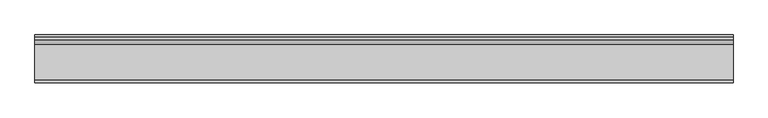
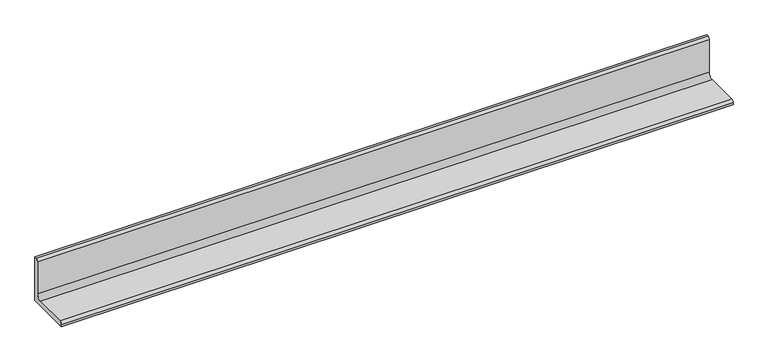
"""IFC4 building model written with IfcOpenShell, lengths in millimetres: beam geometry, NLRS_28_SF_LIB_stalen ligger hoekprofiel gelijkzijdig-AV-MMBS-SRP_gen_rsf : stalen ligger gelijkzijdig hoekprofiel LEQU_gen__150x150x15."""

import ifcopenshell
import ifcopenshell.guid

model = None  # the IFC model being written
_history = None  # IfcOwnerHistory: only IFC2X3 demands one
_inside = {}  # id of a spatial element -> (the spatial element, [elements in it])
_under = {}  # id of a project, library or spatial element -> (it, [spatial elements below it])
_declared = {}  # id of a project -> (the project, [libraries it declares])
_typed = {}  # id of a type object -> (the type object, [elements of that type])
_made_of = {}  # id of a material, layer set ... -> (it, [elements and type objects made of it])


def new_model(schema):
    """Start an empty IFC model of exactly this schema.

    Asked for "IFC4X3", IfcOpenShell would pick the latest addendum, in which some entities
    have other attributes; the version numbers below select the first issue.
    IFC2X3 requires an IfcOwnerHistory on every rooted entity: one is made here for all.
    """
    global model, _history
    if schema == "IFC4X3":
        model = ifcopenshell.file(schema_version=(4, 3, 0, 0))
    else:
        model = ifcopenshell.file(schema=schema)
    _inside.clear()
    _under.clear()
    _declared.clear()
    _typed.clear()
    _made_of.clear()
    _history = None
    if model.schema == "IFC2X3":
        org = make("IfcOrganization", Name="unknown")
        user = make(
            "IfcPersonAndOrganization",
            ThePerson=make("IfcPerson", FamilyName="unknown"),
            TheOrganization=org,
        )
        app = make(
            "IfcApplication",
            ApplicationDeveloper=org,
            Version="unknown",
            ApplicationFullName="unknown",
            ApplicationIdentifier="unknown",
        )
        _history = make(
            "IfcOwnerHistory",
            OwningUser=user,
            OwningApplication=app,
            ChangeAction="ADDED",
            CreationDate=0,
        )
    return model


def make(cls, **values):
    """One entity of the class cls with the attributes given. An attribute that is None is left unset."""
    return model.create_entity(
        cls, **{name: value for name, value in values.items() if value is not None}
    )


def rooted(cls, **values):
    """An entity with a GlobalId (a new one), such as an element, a storey or a relation."""
    return make(cls, GlobalId=ifcopenshell.guid.new(), OwnerHistory=_history, **values)


def si_unit(unit_type, name, prefix=None):
    """IfcSIUnit, for example si_unit("LENGTHUNIT", "METRE", prefix="MILLI")."""
    return make("IfcSIUnit", UnitType=unit_type, Prefix=prefix, Name=name)


def assignment(units):
    """IfcUnitAssignment: the units of a project."""
    return None if units is None else make("IfcUnitAssignment", Units=units)


def point(xyz):
    """IfcCartesianPoint."""
    return None if xyz is None else make("IfcCartesianPoint", Coordinates=xyz)


def direction(xyz):
    """IfcDirection."""
    return None if xyz is None else make("IfcDirection", DirectionRatios=xyz)


def frame(location, z_axis=None, x_axis=None):
    """IfcAxis2Placement3D, a coordinate frame: its origin and axes. An axis left out is left unset."""
    return make(
        "IfcAxis2Placement3D",
        Location=point(location),
        Axis=direction(z_axis),
        RefDirection=direction(x_axis),
    )


def frame_2d(location, x_axis=None):
    """IfcAxis2Placement2D, a coordinate frame in the plane: its origin and x axis."""
    return make(
        "IfcAxis2Placement2D", Location=point(location), RefDirection=direction(x_axis)
    )


def origin():
    """The frame at (0, 0, 0) with its axes left unset."""
    return frame((0.0, 0.0, 0.0))


def place(relative_to, where):
    """IfcLocalPlacement: puts the frame where relative to a parent placement (None: the world)."""
    return make(
        "IfcLocalPlacement", PlacementRelTo=relative_to, RelativePlacement=where
    )


def context(
    kind, dimensions, precision=None, world=None, true_north=None, identifier=None
):
    """IfcGeometricRepresentationContext, for example the 3D "Model" context."""
    return make(
        "IfcGeometricRepresentationContext",
        ContextIdentifier=identifier,
        ContextType=kind,
        CoordinateSpaceDimension=dimensions,
        Precision=precision,
        WorldCoordinateSystem=world,
        TrueNorth=true_north,
    )


def project(units=None, contexts=None):
    """IfcProject with its units and contexts."""
    return rooted(
        "IfcProject",
        Name="project",
        RepresentationContexts=contexts,
        UnitsInContext=assignment(units),
    )


def spatial(cls, under=None, at=None, **own):
    """A site, building, storey or space (cls), placed at a placement, below another one or the project."""
    s = rooted(cls, ObjectPlacement=at, **own)
    if under is not None:
        _under.setdefault(under.id(), (under, []))[1].append(s)
    return s


def polyline(points):
    """IfcPolyline through the points."""
    return make("IfcPolyline", Points=[point(p) for p in points])


def circle_curve(where, radius):
    """IfcCircle in the frame where."""
    return make("IfcCircle", Position=where, Radius=radius)


def trimmed(basis, trim1, trim2, sense, master):
    """IfcTrimmedCurve: the piece of a basis curve between two trims."""
    return make(
        "IfcTrimmedCurve",
        BasisCurve=basis,
        Trim1=trim1,
        Trim2=trim2,
        SenseAgreement=sense,
        MasterRepresentation=master,
    )


def segment(curve, same_sense, transition):
    """IfcCompositeCurveSegment."""
    return make(
        "IfcCompositeCurveSegment",
        Transition=transition,
        SameSense=same_sense,
        ParentCurve=curve,
    )


def composite_curve(segments, self_intersect=None):
    """IfcCompositeCurve: segments joined end to end."""
    return make("IfcCompositeCurve", Segments=segments, SelfIntersect=self_intersect)


def outline(outer, holes=None, kind="AREA"):
    """IfcArbitraryClosedProfileDef: a profile drawn as a closed curve; with holes, ...WithVoids."""
    if holes is None:
        return make("IfcArbitraryClosedProfileDef", ProfileType=kind, OuterCurve=outer)
    return make(
        "IfcArbitraryProfileDefWithVoids",
        ProfileType=kind,
        OuterCurve=outer,
        InnerCurves=holes,
    )


def extrude(swept, where, along, depth):
    """IfcExtrudedAreaSolid: the profile swept, set in the frame where, extruded along a direction by depth."""
    return make(
        "IfcExtrudedAreaSolid",
        SweptArea=swept,
        Position=where,
        ExtrudedDirection=direction(along),
        Depth=depth,
    )


def shape(context_of_items, identifier, shape_type, items):
    """IfcShapeRepresentation: the items that make up one representation, for example the "Body"."""
    return make(
        "IfcShapeRepresentation",
        ContextOfItems=context_of_items,
        RepresentationIdentifier=identifier,
        RepresentationType=shape_type,
        Items=items,
    )


def source(mapping_origin, context_of_items, identifier, shape_type, items):
    """IfcRepresentationMap: a shape defined once, which mapped items show again and again."""
    return make(
        "IfcRepresentationMap",
        MappingOrigin=mapping_origin,
        MappedRepresentation=shape(context_of_items, identifier, shape_type, items),
    )


def transform(
    local_origin,
    x_axis=None,
    y_axis=None,
    z_axis=None,
    scale=None,
    scale2=None,
    scale3=None,
    uniform=True,
):
    """IfcCartesianTransformationOperator3D, or its non-uniform kind. x_axis, y_axis, z_axis: its Axis1, 2, 3."""
    if uniform:
        return make(
            "IfcCartesianTransformationOperator3D",
            Axis1=direction(x_axis),
            Axis2=direction(y_axis),
            LocalOrigin=point(local_origin),
            Scale=scale,
            Axis3=direction(z_axis),
        )
    return make(
        "IfcCartesianTransformationOperator3DnonUniform",
        Axis1=direction(x_axis),
        Axis2=direction(y_axis),
        LocalOrigin=point(local_origin),
        Scale=scale,
        Axis3=direction(z_axis),
        Scale2=scale2,
        Scale3=scale3,
    )


def mapped(mapping_source, mapping_target):
    """IfcMappedItem: shows the shape of a source again, moved by a transform."""
    return make(
        "IfcMappedItem", MappingSource=mapping_source, MappingTarget=mapping_target
    )


def made_of(thing, what):
    """Note that an element or type object is made of a material, layer set ...; save() writes the relation."""
    if what is not None:
        _made_of.setdefault(what.id(), (what, []))[1].append(thing)
    return thing


def element(
    cls,
    number,
    at=None,
    inside=None,
    cuts=None,
    type_object=None,
    material=None,
    context=None,
    identifier="Body",
    shape_type=None,
    held_by="IfcProductDefinitionShape",
    body=None,
    shapes=None,
    **own,
):
    """One element of the class cls, such as IfcWall. Its Tag is "e" and its number.

    at: its placement. inside: the storey or other place that contains it. cuts: it is an
    opening in that element (IfcRelVoidsElement). A single representation is given by context,
    identifier, shape_type and body (its items); several are given by shapes. held_by: the class
    of the entity that holds the representations. save() writes the other relations.
    """
    e = rooted(cls, Tag="e%d" % number, ObjectPlacement=at, **own)
    if body is not None:
        shapes = [shape(context, identifier, shape_type, body)]
    if shapes is not None:
        e.Representation = make(held_by, Representations=shapes)
    if inside is not None:
        _inside.setdefault(inside.id(), (inside, []))[1].append(e)
    if cuts is not None:
        rooted(
            "IfcRelVoidsElement", RelatingBuildingElement=cuts, RelatedOpeningElement=e
        )
    if type_object is not None:
        _typed.setdefault(type_object.id(), (type_object, []))[1].append(e)
    return made_of(e, material)


def aggregate(whole, parts):
    """IfcRelAggregates: a whole, such as a stair, and the parts it consists of."""
    return rooted("IfcRelAggregates", RelatingObject=whole, RelatedObjects=parts)


def save(model, path):
    """Write the relations noted so far, then the file.

    IfcRelAggregates (storeys below a building ...), IfcRelContainedInSpatialStructure (elements
    in a storey), IfcRelDefinesByType, IfcRelAssociatesMaterial and IfcRelDeclares: one each for
    every whole, place, type object, material and project.
    """
    for whole, parts in _under.values():
        aggregate(whole, parts)
    for where, things in _inside.values():
        rooted(
            "IfcRelContainedInSpatialStructure",
            RelatedElements=things,
            RelatingStructure=where,
        )
    for kind, things in _typed.values():
        rooted("IfcRelDefinesByType", RelatedObjects=things, RelatingType=kind)
    for what, things in _made_of.values():
        rooted("IfcRelAssociatesMaterial", RelatedObjects=things, RelatingMaterial=what)
    for by, libraries in _declared.values():
        rooted("IfcRelDeclares", RelatingContext=by, RelatedDefinitions=libraries)
    model.write(path)


def beam_a9a0024c(model_context):
    return source(origin(), model_context, "Body", "SweptSolid", [
        extrude(outline(composite_curve([segment(polyline([(42.5, -42.5), (-107.5, -42.5), (-107.5, -35.5)]), True, "CONTINUOUS"), segment(trimmed(circle_curve(frame_2d((-99.5, -35.5)), 8.0), [point((-107.5, -35.5))], [point((-99.5, -27.5))], False, "CARTESIAN"), True, "CONTINUOUS"), segment(polyline([(-99.5, -27.5), (11.5, -27.5)]), True, "CONTINUOUS"), segment(trimmed(circle_curve(frame_2d((11.5, -11.5)), 16.0), [point((11.5, -27.5))], [point((27.5, -11.5))], True, "CARTESIAN"), True, "CONTINUOUS"), segment(polyline([(27.5, -11.5), (27.5, 99.5)]), True, "CONTINUOUS"), segment(trimmed(circle_curve(frame_2d((35.5, 99.5)), 8.0), [point((27.5, 99.5))], [point((35.5, 107.5))], False, "CARTESIAN"), True, "CONTINUOUS"), segment(polyline([(35.5, 107.5), (42.5, 107.5), (42.5, -42.5)]), True, "CONTINUOUS")], self_intersect=False)), frame((-1095.0, 0.0, 0.0), z_axis=(1.0, 0.0, 0.0), x_axis=(0.0, 1.0, 0.0)), (0.0, 0.0, 1.0), 2190.0),
    ])


if __name__ == "__main__":
    model = new_model("IFC4")
    model_context = context("Model", 3, world=origin())
    ifc_project = project(units=[si_unit("LENGTHUNIT", "METRE", prefix="MILLI")], contexts=[model_context])
    site = spatial("IfcSite", under=ifc_project)
    building = spatial("IfcBuilding", under=site)
    placement = place(None, origin())
    beam_shape = beam_a9a0024c(model_context)
    element("IfcBeam", 1, ObjectType="NLRS_28_SF_LIB_stalen ligger hoekprofiel gelijkzijdig-AV-MMBS-SRP_gen_rsf : stalen ligger gelijkzijdig hoekprofiel LEQU_gen__150x150x15", at=placement, inside=building, context=model_context, shape_type="MappedRepresentation", body=[
        mapped(beam_shape, transform((0.0, 0.0, 0.0), x_axis=(1.0, 0.0, 0.0), y_axis=(0.0, 1.0, 0.0), z_axis=(0.0, 0.0, 1.0))),
    ])
    save(model, "model.ifc")

# Revit data of these elements
# Type "NLRS_28_SF_LIB_stalen ligger hoekprofiel gelijkzijdig-AV-MMBS-SRP_gen_rsf : stalen ligger gelijkzijdig hoekprofiel LEQU_gen__150x150x15"
#   Export Type to IFC As = "IfcBeamType"
#   Type IfcGUID = "2CEqVLPNH8KRN7ghwV3a1U"
#   Type Comments = "L150x150x15"
#   Model = " "
#   Manufacturer = " "
#   Fire Rating = " "
#   Description = "stalen ligger L150x150x15"
#   Assembly Code = "28.11"
#   vz = 107.5 mm
#   vy = 107.5 mm
#   tw = 15 mm
#   tf = 15 mm
#   ri = 8 mm
#   ra = 16 mm
#   d = 150 mm
#   bf = 150 mm
#   NLRS_C_lengte [instance default] = 1524 mm
#   Length [instance default] = 1524 mm
#   Structural Material = NLRS_h2_staal_gen_rsf
#   Keynote = ""
# Element 1 (IfcBeam, "NLRS_28_SF_LIB_stalen ligger hoekprofiel gelijkzijdig-AV-MMBS-SRP_gen_rsf : stalen ligger gelijkzijdig hoekprofiel LEQU_gen__150x150x15")
#   NLRS_C_lengte = 2190 mm
#   Materials on its faces: "NLRS_h2_staal_gen_rsf"
# Materials
#   "NLRS_h2_staal_gen_rsf": class "H - Metaal", colour RGB 189 187 185, transparency 0, Keynote = "h2", Manufacturer = "Revit Standards Foundation", URL = "www.revitstandards.org", Description = "staal", Cost = 0
